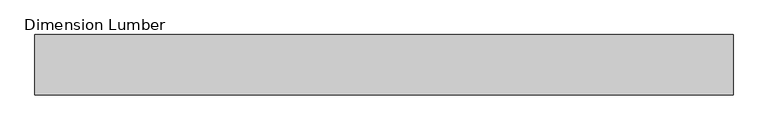
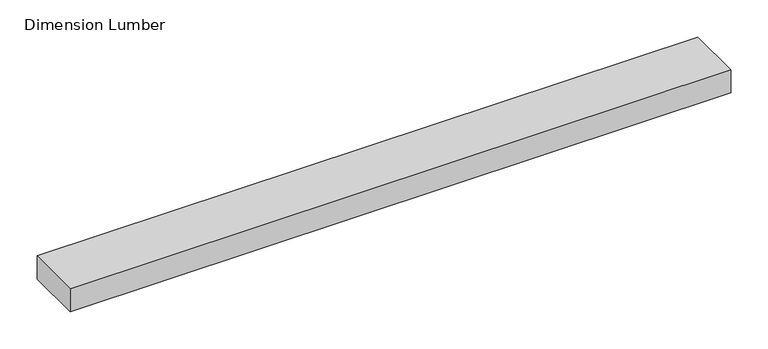
"""IFC4 building model written with IfcOpenShell, lengths in millimetres: beam geometry, Dimension Lumber : Top Supporting Lumbers."""

from ifc_helpers import new_model, si_unit, frame, origin, place, context, project, spatial, polyline, outline, extrude, source, transform, mapped, element, save


def dimension_lumber_dd19c813(model_context):
    return source(origin(), model_context, "Body", "SweptSolid", [
        extrude(outline(polyline([(558.8, 44.45), (558.8, -44.45), (-469.9, -44.45), (-469.9, 44.45), (558.8, 44.45)])), frame((0.0, 0.0, -19.05), z_axis=(0.0, 0.0, 1.0), x_axis=(1.0, 0.0, 0.0)), (0.0, 0.0, 1.0), 38.1),
    ])


if __name__ == "__main__":
    model = new_model("IFC4")
    model_context = context("Model", 3, world=origin())
    ifc_project = project(units=[si_unit("LENGTHUNIT", "METRE", prefix="MILLI")], contexts=[model_context])
    site = spatial("IfcSite", under=ifc_project)
    building = spatial("IfcBuilding", under=site)
    placement = place(None, origin())
    dimension_lumber_shape = dimension_lumber_dd19c813(model_context)
    element("IfcBeam", 1, ObjectType="Dimension Lumber : Top Supporting Lumbers", at=placement, inside=building, context=model_context, shape_type="MappedRepresentation", body=[
        mapped(dimension_lumber_shape, transform((0.0, 0.0, 0.0), x_axis=(1.0, 0.0, 0.0), y_axis=(0.0, 1.0, 0.0), z_axis=(0.0, 0.0, 1.0))),
    ])
    save(model, "model.ifc")

# Revit data of these elements
# Type "Dimension Lumber : Top Supporting Lumbers"
#   Assembly Code = "B10"
#   A = 0.0364583 SF
#   Length [instance default] = 5' - 0"
#   b = 0' - 3 1/2"
#   d = 0' - 1 1/2"
#   Structural Material [instance default] = Softwood, Lumber
# Element 1 (IfcBeam, "Dimension Lumber : Top Supporting Lumbers")
#   Structural Material = Douglas Fir #2
#   Materials on its faces: "Douglas Fir #2"
# Materials
#   "Softwood, Lumber": class "Wood", colour RGB 223 192 134, transparency 0, Description = "Pinus Echinata", Cost = 0
#   "Douglas Fir #2": class "Wood", colour RGB 223 192 134, transparency 0, Description = "Pinus Echinata", Cost = 0
